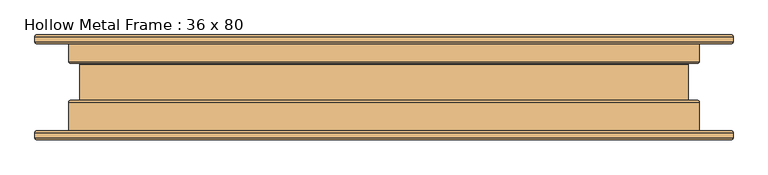
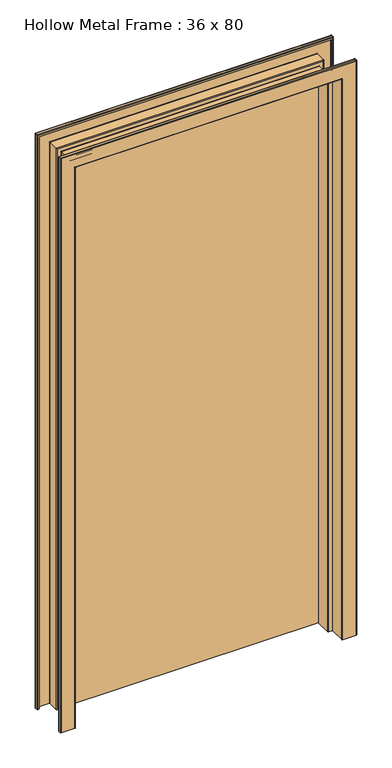
"""IFC4 building model written with IfcOpenShell, lengths in millimetres: door geometry, Hollow Metal Frame : 36 x 80."""

from ifc_helpers import new_model, si_unit, frame, origin, origin_with_axes, place, context, project, spatial, polyline, circle_curve, ellipse_curve, outline, extrude, source, transform, mapped, element, save
from ifc_brep_helpers import plane_surface, cylinder_surface, revolved_surface, advanced_brep


def hollow_metal_frame_36_x_80_ba635d64(model_context):
    return source(origin(), model_context, "Body", "SolidModel", [
        advanced_brep(
        [(-505.42825, -63.5635, 0.0), (-500.0625, -63.5635, 0.0), (-500.0625, -65.11925, 0.0), (-505.42825, -65.11925, 0.0), (-506.44425, -66.13525, 0.0), (-506.44425, -73.66, 0.0), (-505.42825, -74.676, 0.0), (-459.77175, -74.676, 0.0), (-458.75575, -73.66, 0.0), (-458.75575, -21.68525, 0.0), (-456.184, -19.1135, 0.0), (-443.89675, -19.1135, 0.0), (-442.88075, -18.0975, 0.0), (-442.88075, 33.6931, 0.0), (-443.89675, 34.7091, 0.0), (-456.184, 34.7091, 0.0), (-458.75575, 37.28085, 0.0), (-458.75575, 73.5965, 0.0), (-459.77175, 74.6125, 0.0), (-505.42825, 74.6125, 0.0), (-506.44425, 73.5965, 0.0), (-506.44425, 66.07175, 0.0), (-505.42825, 65.05575, 0.0), (-500.0625, 65.05575, 0.0), (-500.0625, 63.5, 0.0), (-505.42825, 63.5, 0.0), (-508.0, 66.07175, 0.0), (-508.0, 73.5965, 0.0), (-505.42825, 76.16825, 0.0), (-459.77175, 76.16825, 0.0), (-457.2, 73.5965, 0.0), (-457.2, 37.28085, 0.0), (-456.184, 36.26485, 0.0), (-443.89675, 36.26485, 0.0), (-441.325, 33.6931, 0.0), (-441.325, -18.0975, 0.0), (-443.89675, -20.66925, 0.0), (-456.184, -20.66925, 0.0), (-457.2, -21.68525, 0.0), (-457.2, -73.66, 0.0), (-459.77175, -76.23175, 0.0), (-505.42825, -76.23175, 0.0), (-508.0, -73.66, 0.0), (-508.0, -66.13525, 0.0), (-508.0, -66.13525, 2082.8000001), (-505.42825, -63.5635, 2080.2282501), (-508.0, -73.66, 2082.8000001), (-505.42825, -76.23175, 2080.2282501), (-459.77175, -76.23175, 2034.5717501), (459.77175, -76.23175, 2034.5717501), (459.77175, -76.23175, 0.0), (505.42825, -76.23175, 0.0), (505.42825, -76.23175, 2080.2282501), (-457.2, -73.66, 2032.0000001), (-457.2, -21.68525, 2032.0000001), (-456.184, -20.66925, 2030.9840001), (-443.89675, -20.66925, 2018.6967501), (443.89675, -20.66925, 2018.6967501), (443.89675, -20.66925, 0.0), (456.184, -20.66925, 0.0), (456.184, -20.66925, 2030.9840001), (-441.325, -18.0975, 2016.1250001), (-441.325, 33.6931, 2016.1250001), (-443.89675, 36.26485, 2018.6967501), (-456.184, 36.26485, 2030.9840001), (456.184, 36.26485, 2030.9840001), (456.184, 36.26485, 0.0), (443.89675, 36.26485, 0.0), (443.89675, 36.26485, 2018.6967501), (-457.2, 37.28085, 2032.0000001), (-457.2, 73.5965, 2032.0000001), (-459.77175, 76.16825, 2034.5717501), (-505.42825, 76.16825, 2080.2282501), (505.42825, 76.16825, 2080.2282501), (505.42825, 76.16825, 0.0), (459.77175, 76.16825, 0.0), (459.77175, 76.16825, 2034.5717501), (-508.0, 73.5965, 2082.8000001), (-508.0, 66.07175, 2082.8000001), (-505.42825, 63.5, 2080.2282501), (-500.0625, 63.5, 2074.8625001), (500.0625, 63.5, 2074.8625001), (500.0625, 63.5, 0.0), (505.42825, 63.5, 0.0), (505.42825, 63.5, 2080.2282501), (-500.0625, 65.05575, 2074.8625001), (-505.42825, 65.05575, 2080.2282501), (505.42825, 65.05575, 2080.2282501), (505.42825, 65.05575, 0.0), (500.0625, 65.05575, 0.0), (500.0625, 65.05575, 2074.8625001), (-506.44425, 66.07175, 2081.2442501), (-506.44425, 73.5965, 2081.2442501), (-505.42825, 74.6125, 2080.2282501), (-459.77175, 74.6125, 2034.5717501), (459.77175, 74.6125, 2034.5717501), (459.77175, 74.6125, 0.0), (505.42825, 74.6125, 0.0), (505.42825, 74.6125, 2080.2282501), (-458.75575, 73.5965, 2033.5557501), (-458.75575, 37.28085, 2033.5557501), (-456.184, 34.7091, 2030.9840001), (-443.89675, 34.7091, 2018.6967501), (443.89675, 34.7091, 2018.6967501), (443.89675, 34.7091, 0.0), (456.184, 34.7091, 0.0), (456.184, 34.7091, 2030.9840001), (-442.88075, 33.6931, 2017.6807501), (-442.88075, -18.0975, 2017.6807501), (-443.89675, -19.1135, 2018.6967501), (-456.184, -19.1135, 2030.9840001), (456.184, -19.1135, 2030.9840001), (456.184, -19.1135, 0.0), (443.89675, -19.1135, 0.0), (443.89675, -19.1135, 2018.6967501), (-458.75575, -21.68525, 2033.5557501), (-458.75575, -73.66, 2033.5557501), (-459.77175, -74.676, 2034.5717501), (-505.42825, -74.676, 2080.2282501), (505.42825, -74.676, 2080.2282501), (505.42825, -74.676, 0.0), (459.77175, -74.676, 0.0), (459.77175, -74.676, 2034.5717501), (-506.44425, -73.66, 2081.2442501), (-506.44425, -66.13525, 2081.2442501), (-505.42825, -65.11925, 2080.2282501), (-500.0625, -65.11925, 2074.8625001), (500.0625, -65.11925, 2074.8625001), (500.0625, -65.11925, 0.0), (505.42825, -65.11925, 0.0), (505.42825, -65.11925, 2080.2282501), (-500.0625, -63.5635, 2074.8625001), (505.42825, -63.5635, 2080.2282501), (505.42825, -63.5635, 0.0), (500.0625, -63.5635, 0.0), (500.0625, -63.5635, 2074.8625001), (508.0, -66.13525, 2082.8000001), (508.0, -73.66, 2082.8000001), (457.2, -73.66, 2032.0000001), (457.2, -21.68525, 2032.0000001), (441.325, -18.0975, 2016.1250001), (441.325, 33.6931, 2016.1250001), (457.2, 37.28085, 2032.0000001), (457.2, 73.5965, 2032.0000001), (508.0, 73.5965, 2082.8000001), (508.0, 66.07175, 2082.8000001), (506.44425, 66.07175, 2081.2442501), (506.44425, 73.5965, 2081.2442501), (458.75575, 73.5965, 2033.5557501), (458.75575, 37.28085, 2033.5557501), (442.88075, 33.6931, 2017.6807501), (442.88075, -18.0975, 2017.6807501), (458.75575, -21.68525, 2033.5557501), (458.75575, -73.66, 2033.5557501), (506.44425, -73.66, 2081.2442501), (506.44425, -66.13525, 2081.2442501), (508.0, -66.13525, 0.0), (508.0, -73.66, 0.0), (457.2, -73.66, 0.0), (457.2, -21.68525, 0.0), (441.325, -18.0975, 0.0), (441.325, 33.6931, 0.0), (457.2, 37.28085, 0.0), (457.2, 73.5965, 0.0), (508.0, 73.5965, 0.0), (508.0, 66.07175, 0.0), (506.44425, 66.07175, 0.0), (506.44425, 73.5965, 0.0), (458.75575, 73.5965, 0.0), (458.75575, 37.28085, 0.0), (442.88075, 33.6931, 0.0), (442.88075, -18.0975, 0.0), (458.75575, -21.68525, 0.0), (458.75575, -73.66, 0.0), (506.44425, -73.66, 0.0), (506.44425, -66.13525, 0.0)],
        [
            (0, 1),
            (1, 2),
            (2, 3),
            (3, 4, circle_curve(frame((-505.42825, -66.13525, 0.0), z_axis=(0.0, 0.0, 1.0), x_axis=(0.0, 1.0, 0.0)), 1.016)),
            (4, 5),
            (5, 6, circle_curve(frame((-505.42825, -73.66, 0.0), z_axis=(0.0, 0.0, 1.0), x_axis=(0.0, 1.0, 0.0)), 1.016)),
            (6, 7),
            (7, 8, circle_curve(frame((-459.77175, -73.66, 0.0), z_axis=(0.0, 0.0, 1.0), x_axis=(0.0, 1.0, 0.0)), 1.016)),
            (8, 9),
            (9, 10, circle_curve(frame((-456.184, -21.68525, 0.0), z_axis=(0.0, 0.0, -1.0), x_axis=(0.0, 1.0, 0.0)), 2.57175)),
            (10, 11),
            (11, 12, circle_curve(frame((-443.89675, -18.0975, 0.0), z_axis=(0.0, 0.0, 1.0), x_axis=(0.0, 1.0, 0.0)), 1.016)),
            (12, 13),
            (13, 14, circle_curve(frame((-443.89675, 33.6931, 0.0), z_axis=(0.0, 0.0, 1.0), x_axis=(0.0, 1.0, 0.0)), 1.016)),
            (14, 15),
            (15, 16, circle_curve(frame((-456.184, 37.28085, 0.0), z_axis=(0.0, 0.0, -1.0), x_axis=(0.0, 1.0, 0.0)), 2.57175)),
            (16, 17),
            (17, 18, circle_curve(frame((-459.77175, 73.5965, 0.0), z_axis=(0.0, 0.0, 1.0), x_axis=(0.0, 1.0, 0.0)), 1.016)),
            (18, 19),
            (19, 20, circle_curve(frame((-505.42825, 73.5965, 0.0), z_axis=(0.0, 0.0, 1.0), x_axis=(0.0, 1.0, 0.0)), 1.016)),
            (20, 21),
            (21, 22, circle_curve(frame((-505.42825, 66.07175, 0.0), z_axis=(0.0, 0.0, 1.0), x_axis=(0.0, 1.0, 0.0)), 1.016)),
            (22, 23),
            (23, 24),
            (24, 25),
            (25, 26, circle_curve(frame((-505.42825, 66.07175, 0.0), z_axis=(0.0, 0.0, -1.0), x_axis=(0.0, 1.0, 0.0)), 2.57175)),
            (26, 27),
            (27, 28, circle_curve(frame((-505.42825, 73.5965, 0.0), z_axis=(0.0, 0.0, -1.0), x_axis=(0.0, 1.0, 0.0)), 2.57175)),
            (28, 29),
            (29, 30, circle_curve(frame((-459.77175, 73.5965, 0.0), z_axis=(0.0, 0.0, -1.0), x_axis=(0.0, 1.0, 0.0)), 2.57175)),
            (30, 31),
            (31, 32, circle_curve(frame((-456.184, 37.28085, 0.0), z_axis=(0.0, 0.0, 1.0), x_axis=(0.0, 1.0, 0.0)), 1.016)),
            (32, 33),
            (33, 34, circle_curve(frame((-443.89675, 33.6931, 0.0), z_axis=(0.0, 0.0, -1.0), x_axis=(0.0, 1.0, 0.0)), 2.57175)),
            (34, 35),
            (35, 36, circle_curve(frame((-443.89675, -18.0975, 0.0), z_axis=(0.0, 0.0, -1.0), x_axis=(0.0, 1.0, 0.0)), 2.57175)),
            (36, 37),
            (37, 38, circle_curve(frame((-456.184, -21.68525, 0.0), z_axis=(0.0, 0.0, 1.0), x_axis=(0.0, 1.0, 0.0)), 1.016)),
            (38, 39),
            (39, 40, circle_curve(frame((-459.77175, -73.66, 0.0), z_axis=(0.0, 0.0, -1.0), x_axis=(0.0, 1.0, 0.0)), 2.57175)),
            (40, 41),
            (41, 42, circle_curve(frame((-505.42825, -73.66, 0.0), z_axis=(0.0, 0.0, -1.0), x_axis=(0.0, 1.0, 0.0)), 2.57175)),
            (42, 43),
            (43, 0, circle_curve(frame((-505.42825, -66.13525, 0.0), z_axis=(0.0, 0.0, -1.0), x_axis=(0.0, 1.0, 0.0)), 2.57175)),
            (43, 44),
            (44, 45, ellipse_curve(frame((-505.42825, -66.13525, 2080.2282501), z_axis=(-0.7071067811865475, 0.0, -0.7071067811865475), x_axis=(0.7071067811865474, 0.0, -0.7071067811865476)), 3.6370037, 2.57175)),
            (45, 0),
            (42, 46),
            (46, 44),
            (41, 47),
            (47, 46, ellipse_curve(frame((-505.42825, -73.66, 2080.2282501), z_axis=(-0.7071067811865475, 0.0, -0.7071067811865475), x_axis=(0.7071067811865474, 0.0, -0.7071067811865476)), 3.6370037, 2.57175)),
            (40, 48),
            (48, 49),
            (49, 50),
            (50, 51),
            (51, 52),
            (52, 47),
            (39, 53),
            (53, 48, ellipse_curve(frame((-459.77175, -73.66, 2034.5717501), z_axis=(-0.7071067811865475, 0.0, -0.7071067811865475), x_axis=(0.7071067811865474, 0.0, -0.7071067811865476)), 3.6370037, 2.57175)),
            (38, 54),
            (54, 53),
            (37, 55),
            (55, 54, ellipse_curve(frame((-456.184, -21.68525, 2030.9840001), z_axis=(0.7071067811865475, 0.0, 0.7071067811865475), x_axis=(-0.7071067811865474, 0.0, 0.7071067811865476)), 1.436841, 1.016)),
            (36, 56),
            (56, 57),
            (57, 58),
            (58, 59),
            (59, 60),
            (60, 55),
            (35, 61),
            (61, 56, ellipse_curve(frame((-443.89675, -18.0975, 2018.6967501), z_axis=(-0.7071067811865475, 0.0, -0.7071067811865475), x_axis=(0.7071067811865474, 0.0, -0.7071067811865476)), 3.6370037, 2.57175)),
            (34, 62),
            (62, 61),
            (33, 63),
            (63, 62, ellipse_curve(frame((-443.89675, 33.6931, 2018.6967501), z_axis=(-0.7071067811865475, 0.0, -0.7071067811865475), x_axis=(0.7071067811865474, 0.0, -0.7071067811865476)), 3.6370037, 2.57175)),
            (32, 64),
            (64, 65),
            (65, 66),
            (66, 67),
            (67, 68),
            (68, 63),
            (31, 69),
            (69, 64, ellipse_curve(frame((-456.184, 37.28085, 2030.9840001), z_axis=(0.7071067811865475, 0.0, 0.7071067811865475), x_axis=(-0.7071067811865474, 0.0, 0.7071067811865476)), 1.436841, 1.016)),
            (30, 70),
            (70, 69),
            (29, 71),
            (71, 70, ellipse_curve(frame((-459.77175, 73.5965, 2034.5717501), z_axis=(-0.7071067811865475, 0.0, -0.7071067811865475), x_axis=(0.7071067811865474, 0.0, -0.7071067811865476)), 3.6370037, 2.57175)),
            (28, 72),
            (72, 73),
            (73, 74),
            (74, 75),
            (75, 76),
            (76, 71),
            (27, 77),
            (77, 72, ellipse_curve(frame((-505.42825, 73.5965, 2080.2282501), z_axis=(-0.7071067811865475, 0.0, -0.7071067811865475), x_axis=(0.7071067811865474, 0.0, -0.7071067811865476)), 3.6370037, 2.57175)),
            (26, 78),
            (78, 77),
            (25, 79),
            (79, 78, ellipse_curve(frame((-505.42825, 66.07175, 2080.2282501), z_axis=(-0.7071067811865475, 0.0, -0.7071067811865475), x_axis=(0.7071067811865474, 0.0, -0.7071067811865476)), 3.6370037, 2.57175)),
            (24, 80),
            (80, 81),
            (81, 82),
            (82, 83),
            (83, 84),
            (84, 79),
            (23, 85),
            (85, 80),
            (22, 86),
            (86, 87),
            (87, 88),
            (88, 89),
            (89, 90),
            (90, 85),
            (21, 91),
            (91, 86, ellipse_curve(frame((-505.42825, 66.07175, 2080.2282501), z_axis=(0.7071067811865475, 0.0, 0.7071067811865475), x_axis=(-0.7071067811865474, 0.0, 0.7071067811865476)), 1.436841, 1.016)),
            (20, 92),
            (92, 91),
            (19, 93),
            (93, 92, ellipse_curve(frame((-505.42825, 73.5965, 2080.2282501), z_axis=(0.7071067811865475, 0.0, 0.7071067811865475), x_axis=(-0.7071067811865474, 0.0, 0.7071067811865476)), 1.436841, 1.016)),
            (18, 94),
            (94, 95),
            (95, 96),
            (96, 97),
            (97, 98),
            (98, 93),
            (17, 99),
            (99, 94, ellipse_curve(frame((-459.77175, 73.5965, 2034.5717501), z_axis=(0.7071067811865475, 0.0, 0.7071067811865475), x_axis=(-0.7071067811865474, 0.0, 0.7071067811865476)), 1.436841, 1.016)),
            (16, 100),
            (100, 99),
            (15, 101),
            (101, 100, ellipse_curve(frame((-456.184, 37.28085, 2030.9840001), z_axis=(-0.7071067811865475, 0.0, -0.7071067811865475), x_axis=(0.7071067811865474, 0.0, -0.7071067811865476)), 3.6370037, 2.57175)),
            (14, 102),
            (102, 103),
            (103, 104),
            (104, 105),
            (105, 106),
            (106, 101),
            (13, 107),
            (107, 102, ellipse_curve(frame((-443.89675, 33.6931, 2018.6967501), z_axis=(0.7071067811865475, 0.0, 0.7071067811865475), x_axis=(-0.7071067811865474, 0.0, 0.7071067811865476)), 1.436841, 1.016)),
            (12, 108),
            (108, 107),
            (11, 109),
            (109, 108, ellipse_curve(frame((-443.89675, -18.0975, 2018.6967501), z_axis=(0.7071067811865475, 0.0, 0.7071067811865475), x_axis=(-0.7071067811865474, 0.0, 0.7071067811865476)), 1.436841, 1.016)),
            (10, 110),
            (110, 111),
            (111, 112),
            (112, 113),
            (113, 114),
            (114, 109),
            (9, 115),
            (115, 110, ellipse_curve(frame((-456.184, -21.68525, 2030.9840001), z_axis=(-0.7071067811865475, 0.0, -0.7071067811865475), x_axis=(0.7071067811865474, 0.0, -0.7071067811865476)), 3.6370037, 2.57175)),
            (8, 116),
            (116, 115),
            (7, 117),
            (117, 116, ellipse_curve(frame((-459.77175, -73.66, 2034.5717501), z_axis=(0.7071067811865475, 0.0, 0.7071067811865475), x_axis=(-0.7071067811865474, 0.0, 0.7071067811865476)), 1.436841, 1.016)),
            (6, 118),
            (118, 119),
            (119, 120),
            (120, 121),
            (121, 122),
            (122, 117),
            (5, 123),
            (123, 118, ellipse_curve(frame((-505.42825, -73.66, 2080.2282501), z_axis=(0.7071067811865475, 0.0, 0.7071067811865475), x_axis=(-0.7071067811865474, 0.0, 0.7071067811865476)), 1.436841, 1.016)),
            (4, 124),
            (124, 123),
            (3, 125),
            (125, 124, ellipse_curve(frame((-505.42825, -66.13525, 2080.2282501), z_axis=(0.7071067811865475, 0.0, 0.7071067811865475), x_axis=(-0.7071067811865474, 0.0, 0.7071067811865476)), 1.436841, 1.016)),
            (2, 126),
            (126, 127),
            (127, 128),
            (128, 129),
            (129, 130),
            (130, 125),
            (1, 131),
            (131, 126),
            (45, 132),
            (132, 133),
            (133, 134),
            (134, 135),
            (135, 131),
            (44, 136),
            (136, 132, ellipse_curve(frame((505.42825, -66.13525, 2080.2282501), z_axis=(-0.7071067811865475, 0.0, 0.7071067811865475), x_axis=(-0.7071067811865476, 0.0, -0.7071067811865474)), 3.6370037, 2.57175)),
            (46, 137),
            (137, 136),
            (52, 137, ellipse_curve(frame((505.42825, -73.66, 2080.2282501), z_axis=(-0.7071067811865475, 0.0, 0.7071067811865475), x_axis=(-0.7071067811865476, 0.0, -0.7071067811865474)), 3.6370037, 2.57175)),
            (53, 138),
            (138, 49, ellipse_curve(frame((459.77175, -73.66, 2034.5717501), z_axis=(-0.7071067811865475, 0.0, 0.7071067811865475), x_axis=(-0.7071067811865476, 0.0, -0.7071067811865474)), 3.6370037, 2.57175)),
            (54, 139),
            (139, 138),
            (60, 139, ellipse_curve(frame((456.184, -21.68525, 2030.9840001), z_axis=(0.7071067811865475, 0.0, -0.7071067811865475), x_axis=(0.7071067811865476, 0.0, 0.7071067811865474)), 1.436841, 1.016)),
            (61, 140),
            (140, 57, ellipse_curve(frame((443.89675, -18.0975, 2018.6967501), z_axis=(-0.7071067811865475, 0.0, 0.7071067811865475), x_axis=(-0.7071067811865476, 0.0, -0.7071067811865474)), 3.6370037, 2.57175)),
            (62, 141),
            (141, 140),
            (68, 141, ellipse_curve(frame((443.89675, 33.6931, 2018.6967501), z_axis=(-0.7071067811865475, 0.0, 0.7071067811865475), x_axis=(-0.7071067811865476, 0.0, -0.7071067811865474)), 3.6370037, 2.57175)),
            (69, 142),
            (142, 65, ellipse_curve(frame((456.184, 37.28085, 2030.9840001), z_axis=(0.7071067811865475, 0.0, -0.7071067811865475), x_axis=(0.7071067811865476, 0.0, 0.7071067811865474)), 1.436841, 1.016)),
            (70, 143),
            (143, 142),
            (76, 143, ellipse_curve(frame((459.77175, 73.5965, 2034.5717501), z_axis=(-0.7071067811865475, 0.0, 0.7071067811865475), x_axis=(-0.7071067811865476, 0.0, -0.7071067811865474)), 3.6370037, 2.57175)),
            (77, 144),
            (144, 73, ellipse_curve(frame((505.42825, 73.5965, 2080.2282501), z_axis=(-0.7071067811865475, 0.0, 0.7071067811865475), x_axis=(-0.7071067811865476, 0.0, -0.7071067811865474)), 3.6370037, 2.57175)),
            (78, 145),
            (145, 144),
            (84, 145, ellipse_curve(frame((505.42825, 66.07175, 2080.2282501), z_axis=(-0.7071067811865475, 0.0, 0.7071067811865475), x_axis=(-0.7071067811865476, 0.0, -0.7071067811865474)), 3.6370037, 2.57175)),
            (90, 81),
            (91, 146),
            (146, 87, ellipse_curve(frame((505.42825, 66.07175, 2080.2282501), z_axis=(0.7071067811865475, 0.0, -0.7071067811865475), x_axis=(0.7071067811865476, 0.0, 0.7071067811865474)), 1.436841, 1.016)),
            (92, 147),
            (147, 146),
            (98, 147, ellipse_curve(frame((505.42825, 73.5965, 2080.2282501), z_axis=(0.7071067811865475, 0.0, -0.7071067811865475), x_axis=(0.7071067811865476, 0.0, 0.7071067811865474)), 1.436841, 1.016)),
            (99, 148),
            (148, 95, ellipse_curve(frame((459.77175, 73.5965, 2034.5717501), z_axis=(0.7071067811865475, 0.0, -0.7071067811865475), x_axis=(0.7071067811865476, 0.0, 0.7071067811865474)), 1.436841, 1.016)),
            (100, 149),
            (149, 148),
            (106, 149, ellipse_curve(frame((456.184, 37.28085, 2030.9840001), z_axis=(-0.7071067811865475, 0.0, 0.7071067811865475), x_axis=(-0.7071067811865476, 0.0, -0.7071067811865474)), 3.6370037, 2.57175)),
            (107, 150),
            (150, 103, ellipse_curve(frame((443.89675, 33.6931, 2018.6967501), z_axis=(0.7071067811865475, 0.0, -0.7071067811865475), x_axis=(0.7071067811865476, 0.0, 0.7071067811865474)), 1.436841, 1.016)),
            (108, 151),
            (151, 150),
            (114, 151, ellipse_curve(frame((443.89675, -18.0975, 2018.6967501), z_axis=(0.7071067811865475, 0.0, -0.7071067811865475), x_axis=(0.7071067811865476, 0.0, 0.7071067811865474)), 1.436841, 1.016)),
            (115, 152),
            (152, 111, ellipse_curve(frame((456.184, -21.68525, 2030.9840001), z_axis=(-0.7071067811865475, 0.0, 0.7071067811865475), x_axis=(-0.7071067811865476, 0.0, -0.7071067811865474)), 3.6370037, 2.57175)),
            (116, 153),
            (153, 152),
            (122, 153, ellipse_curve(frame((459.77175, -73.66, 2034.5717501), z_axis=(0.7071067811865475, 0.0, -0.7071067811865475), x_axis=(0.7071067811865476, 0.0, 0.7071067811865474)), 1.436841, 1.016)),
            (123, 154),
            (154, 119, ellipse_curve(frame((505.42825, -73.66, 2080.2282501), z_axis=(0.7071067811865475, 0.0, -0.7071067811865475), x_axis=(0.7071067811865476, 0.0, 0.7071067811865474)), 1.436841, 1.016)),
            (124, 155),
            (155, 154),
            (130, 155, ellipse_curve(frame((505.42825, -66.13525, 2080.2282501), z_axis=(0.7071067811865475, 0.0, -0.7071067811865475), x_axis=(0.7071067811865476, 0.0, 0.7071067811865474)), 1.436841, 1.016)),
            (135, 127),
            (133, 156, circle_curve(frame((505.42825, -66.13525, 0.0), z_axis=(0.0, 0.0, -1.0), x_axis=(0.0, 1.0, 0.0)), 2.57175)),
            (156, 157),
            (157, 51, circle_curve(frame((505.42825, -73.66, 0.0), z_axis=(0.0, 0.0, -1.0), x_axis=(0.0, 1.0, 0.0)), 2.57175)),
            (50, 158, circle_curve(frame((459.77175, -73.66, 0.0), z_axis=(0.0, 0.0, -1.0), x_axis=(0.0, 1.0, 0.0)), 2.57175)),
            (158, 159),
            (159, 59, circle_curve(frame((456.184, -21.68525, 0.0), z_axis=(0.0, 0.0, 1.0), x_axis=(0.0, 1.0, 0.0)), 1.016)),
            (58, 160, circle_curve(frame((443.89675, -18.0975, 0.0), z_axis=(0.0, 0.0, -1.0), x_axis=(0.0, 1.0, 0.0)), 2.57175)),
            (160, 161),
            (161, 67, circle_curve(frame((443.89675, 33.6931, 0.0), z_axis=(0.0, 0.0, -1.0), x_axis=(0.0, 1.0, 0.0)), 2.57175)),
            (66, 162, circle_curve(frame((456.184, 37.28085, 0.0), z_axis=(0.0, 0.0, 1.0), x_axis=(0.0, 1.0, 0.0)), 1.016)),
            (162, 163),
            (163, 75, circle_curve(frame((459.77175, 73.5965, 0.0), z_axis=(0.0, 0.0, -1.0), x_axis=(0.0, 1.0, 0.0)), 2.57175)),
            (74, 164, circle_curve(frame((505.42825, 73.5965, 0.0), z_axis=(0.0, 0.0, -1.0), x_axis=(0.0, 1.0, 0.0)), 2.57175)),
            (164, 165),
            (165, 83, circle_curve(frame((505.42825, 66.07175, 0.0), z_axis=(0.0, 0.0, -1.0), x_axis=(0.0, 1.0, 0.0)), 2.57175)),
            (82, 89),
            (88, 166, circle_curve(frame((505.42825, 66.07175, 0.0), z_axis=(0.0, 0.0, 1.0), x_axis=(0.0, 1.0, 0.0)), 1.016)),
            (166, 167),
            (167, 97, circle_curve(frame((505.42825, 73.5965, 0.0), z_axis=(0.0, 0.0, 1.0), x_axis=(0.0, 1.0, 0.0)), 1.016)),
            (96, 168, circle_curve(frame((459.77175, 73.5965, 0.0), z_axis=(0.0, 0.0, 1.0), x_axis=(0.0, 1.0, 0.0)), 1.016)),
            (168, 169),
            (169, 105, circle_curve(frame((456.184, 37.28085, 0.0), z_axis=(0.0, 0.0, -1.0), x_axis=(0.0, 1.0, 0.0)), 2.57175)),
            (104, 170, circle_curve(frame((443.89675, 33.6931, 0.0), z_axis=(0.0, 0.0, 1.0), x_axis=(0.0, 1.0, 0.0)), 1.016)),
            (170, 171),
            (171, 113, circle_curve(frame((443.89675, -18.0975, 0.0), z_axis=(0.0, 0.0, 1.0), x_axis=(0.0, 1.0, 0.0)), 1.016)),
            (112, 172, circle_curve(frame((456.184, -21.68525, 0.0), z_axis=(0.0, 0.0, -1.0), x_axis=(0.0, 1.0, 0.0)), 2.57175)),
            (172, 173),
            (173, 121, circle_curve(frame((459.77175, -73.66, 0.0), z_axis=(0.0, 0.0, 1.0), x_axis=(0.0, 1.0, 0.0)), 1.016)),
            (120, 174, circle_curve(frame((505.42825, -73.66, 0.0), z_axis=(0.0, 0.0, 1.0), x_axis=(0.0, 1.0, 0.0)), 1.016)),
            (174, 175),
            (175, 129, circle_curve(frame((505.42825, -66.13525, 0.0), z_axis=(0.0, 0.0, 1.0), x_axis=(0.0, 1.0, 0.0)), 1.016)),
            (128, 134),
            (136, 156),
            (137, 157),
            (138, 158),
            (139, 159),
            (140, 160),
            (141, 161),
            (142, 162),
            (143, 163),
            (144, 164),
            (145, 165),
            (146, 166),
            (147, 167),
            (148, 168),
            (149, 169),
            (150, 170),
            (151, 171),
            (152, 172),
            (153, 173),
            (154, 174),
            (155, 175),
        ],
        [
            plane_surface(frame((-468.3125, 63.5, 0.0), z_axis=(0.0, 0.0, -1.0), x_axis=(1.0, 0.0, 0.0))),
            cylinder_surface(frame((-505.42825, -66.13525, 0.0), z_axis=(0.0, 0.0, -1.0), x_axis=(0.0, 1.0, 0.0)), 2.57175),
            plane_surface(frame((-508.0, -66.13525, 0.0), z_axis=(-1.0, 0.0, 0.0), x_axis=(0.0, 0.0, 1.0))),
            cylinder_surface(frame((-505.42825, -73.66, 0.0), z_axis=(0.0, 0.0, -1.0), x_axis=(0.0, 1.0, 0.0)), 2.57175),
            plane_surface(frame((-505.42825, -76.23175, 0.0), z_axis=(0.0, -1.0, 0.0), x_axis=(0.0, 0.0, 1.0))),
            cylinder_surface(frame((-459.77175, -73.66, 0.0), z_axis=(0.0, 0.0, -1.0), x_axis=(0.0, 1.0, 0.0)), 2.57175),
            plane_surface(frame((-457.2, -73.66, 0.0), z_axis=(1.0, 0.0, 0.0), x_axis=(0.0, 0.0, 1.0))),
            revolved_surface(polyline([(-456.184, -20.669249999999998, 2032.0000001145868), (-456.184, -20.669249999999998, 0.0)]), (-456.184, -21.68525, 0.0), (0.0, 0.0, 1.0)),
            plane_surface(frame((-456.184, -20.66925, 0.0), z_axis=(0.0, -1.0, 0.0), x_axis=(0.0, 0.0, 1.0))),
            cylinder_surface(frame((-443.89675, -18.0975, 0.0), z_axis=(0.0, 0.0, -1.0), x_axis=(0.0, 1.0, 0.0)), 2.57175),
            plane_surface(frame((-441.325, -18.0975, 0.0), z_axis=(1.0, 0.0, 0.0), x_axis=(0.0, 0.0, 1.0))),
            cylinder_surface(frame((-443.89675, 33.6931, 0.0), z_axis=(0.0, 0.0, -1.0), x_axis=(0.0, 1.0, 0.0)), 2.57175),
            plane_surface(frame((-443.89675, 36.26485, 0.0), z_axis=(0.0, 1.0, 0.0), x_axis=(0.0, 0.0, 1.0))),
            revolved_surface(polyline([(-456.184, 38.29685, 2032.0000001145868), (-456.184, 38.29685, 0.0)]), (-456.184, 37.28085, 0.0), (0.0, 0.0, 1.0)),
            plane_surface(frame((-457.2, 37.28085, 0.0), z_axis=(1.0, 0.0, 0.0), x_axis=(0.0, 0.0, 1.0))),
            cylinder_surface(frame((-459.77175, 73.5965, 0.0), z_axis=(0.0, 0.0, -1.0), x_axis=(0.0, 1.0, 0.0)), 2.57175),
            plane_surface(frame((-459.77175, 76.16825, 0.0), z_axis=(0.0, 1.0, 0.0), x_axis=(0.0, 0.0, 1.0))),
            cylinder_surface(frame((-505.42825, 73.5965, 0.0), z_axis=(0.0, 0.0, -1.0), x_axis=(0.0, 1.0, 0.0)), 2.57175),
            plane_surface(frame((-508.0, 73.5965, 0.0), z_axis=(-1.0, 0.0, 0.0), x_axis=(0.0, 0.0, 1.0))),
            cylinder_surface(frame((-505.42825, 66.07175, 0.0), z_axis=(0.0, 0.0, -1.0), x_axis=(0.0, 1.0, 0.0)), 2.57175),
            plane_surface(frame((-505.42825, 63.5, 0.0), z_axis=(0.0, -1.0, 0.0), x_axis=(0.0, 0.0, 1.0))),
            plane_surface(frame((-500.0625, 63.5, 0.0), z_axis=(1.0, 0.0, 0.0), x_axis=(0.0, 0.0, 1.0))),
            plane_surface(frame((-500.0625, 65.05575, 0.0), z_axis=(0.0, 1.0, 0.0), x_axis=(0.0, 0.0, 1.0))),
            revolved_surface(polyline([(-505.42825, 67.08775, 2081.244250114587), (-505.42825, 67.08775, 0.0)]), (-505.42825, 66.07175, 0.0), (0.0, 0.0, 1.0)),
            plane_surface(frame((-506.44425, 66.07175, 0.0), z_axis=(1.0, 0.0, 0.0), x_axis=(0.0, 0.0, 1.0))),
            revolved_surface(polyline([(-505.42825, 74.61250000000001, 2081.244250114587), (-505.42825, 74.61250000000001, 0.0)]), (-505.42825, 73.5965, 0.0), (0.0, 0.0, 1.0)),
            plane_surface(frame((-505.42825, 74.6125, 0.0), z_axis=(0.0, -1.0, 0.0), x_axis=(0.0, 0.0, 1.0))),
            revolved_surface(polyline([(-459.77175, 74.61250000000001, 2035.5877501145867), (-459.77175, 74.61250000000001, 0.0)]), (-459.77175, 73.5965, 0.0), (0.0, 0.0, 1.0)),
            plane_surface(frame((-458.75575, 73.5965, 0.0), z_axis=(-1.0, 0.0, 0.0), x_axis=(0.0, 0.0, 1.0))),
            cylinder_surface(frame((-456.184, 37.28085, 0.0), z_axis=(0.0, 0.0, -1.0), x_axis=(0.0, 1.0, 0.0)), 2.57175),
            plane_surface(frame((-456.184, 34.7091, 0.0), z_axis=(0.0, -1.0, 0.0), x_axis=(0.0, 0.0, 1.0))),
            revolved_surface(polyline([(-443.89675, 34.7091, 2019.7127501145867), (-443.89675, 34.7091, 0.0)]), (-443.89675, 33.6931, 0.0), (0.0, 0.0, 1.0)),
            plane_surface(frame((-442.88075, 33.6931, 0.0), z_axis=(-1.0, 0.0, 0.0), x_axis=(0.0, 0.0, 1.0))),
            revolved_surface(polyline([(-443.89675, -17.0815, 2019.7127501145867), (-443.89675, -17.0815, 0.0)]), (-443.89675, -18.0975, 0.0), (0.0, 0.0, 1.0)),
            plane_surface(frame((-443.89675, -19.1135, 0.0), z_axis=(0.0, 1.0, 0.0), x_axis=(0.0, 0.0, 1.0))),
            cylinder_surface(frame((-456.184, -21.68525, 0.0), z_axis=(0.0, 0.0, -1.0), x_axis=(0.0, 1.0, 0.0)), 2.57175),
            plane_surface(frame((-458.75575, -21.68525, 0.0), z_axis=(-1.0, 0.0, 0.0), x_axis=(0.0, 0.0, 1.0))),
            revolved_surface(polyline([(-459.77175, -72.64399999999999, 2035.5877501145867), (-459.77175, -72.64399999999999, 0.0)]), (-459.77175, -73.66, 0.0), (0.0, 0.0, 1.0)),
            plane_surface(frame((-459.77175, -74.676, 0.0), z_axis=(0.0, 1.0, 0.0), x_axis=(0.0, 0.0, 1.0))),
            revolved_surface(polyline([(-505.42825, -72.64399999999999, 2081.244250114587), (-505.42825, -72.64399999999999, 0.0)]), (-505.42825, -73.66, 0.0), (0.0, 0.0, 1.0)),
            plane_surface(frame((-506.44425, -73.66, 0.0), z_axis=(1.0, 0.0, 0.0), x_axis=(0.0, 0.0, 1.0))),
            revolved_surface(polyline([(-505.42825, -65.11925, 2081.244250114587), (-505.42825, -65.11925, 0.0)]), (-505.42825, -66.13525, 0.0), (0.0, 0.0, 1.0)),
            plane_surface(frame((-505.42825, -65.11925, 0.0), z_axis=(0.0, -1.0, 0.0), x_axis=(0.0, 0.0, 1.0))),
            plane_surface(frame((-500.0625, -65.11925, 0.0), z_axis=(1.0, 0.0, 0.0), x_axis=(0.0, 0.0, 1.0))),
            plane_surface(frame((-500.0625, -63.5635, 0.0), z_axis=(0.0, 1.0, 0.0), x_axis=(0.0, 0.0, 1.0))),
            cylinder_surface(frame((-468.3125, -66.13525, 2080.2282501), z_axis=(-1.0, 0.0, 0.0), x_axis=(0.0, 1.0, 0.0)), 2.57175),
            plane_surface(frame((-508.0, -66.13525, 2082.8000001), z_axis=(0.0, 0.0, 1.0), x_axis=(1.0, 0.0, 0.0))),
            cylinder_surface(frame((-468.3125, -73.66, 2080.2282501), z_axis=(-1.0, 0.0, 0.0), x_axis=(0.0, 1.0, 0.0)), 2.57175),
            cylinder_surface(frame((-468.3125, -73.66, 2034.5717501), z_axis=(-1.0, 0.0, 0.0), x_axis=(0.0, 1.0, 0.0)), 2.57175),
            plane_surface(frame((-457.2, -73.66, 2032.0000001), z_axis=(0.0, 0.0, -1.0), x_axis=(1.0, 0.0, 0.0))),
            revolved_surface(polyline([(457.20000001458686, -20.669249999999998, 2030.9840001), (-457.20000001458686, -20.669249999999998, 2030.9840001)]), (-468.3125, -21.68525, 2030.9840001), (1.0, 0.0, 0.0)),
            cylinder_surface(frame((-468.3125, -18.0975, 2018.6967501), z_axis=(-1.0, 0.0, 0.0), x_axis=(0.0, 1.0, 0.0)), 2.57175),
            plane_surface(frame((-441.325, -18.0975, 2016.1250001), z_axis=(0.0, 0.0, -1.0), x_axis=(1.0, 0.0, 0.0))),
            cylinder_surface(frame((-468.3125, 33.6931, 2018.6967501), z_axis=(-1.0, 0.0, 0.0), x_axis=(0.0, 1.0, 0.0)), 2.57175),
            revolved_surface(polyline([(457.20000001458686, 38.29685, 2030.9840001), (-457.20000001458686, 38.29685, 2030.9840001)]), (-468.3125, 37.28085, 2030.9840001), (1.0, 0.0, 0.0)),
            plane_surface(frame((-457.2, 37.28085, 2032.0000001), z_axis=(0.0, 0.0, -1.0), x_axis=(1.0, 0.0, 0.0))),
            cylinder_surface(frame((-468.3125, 73.5965, 2034.5717501), z_axis=(-1.0, 0.0, 0.0), x_axis=(0.0, 1.0, 0.0)), 2.57175),
            cylinder_surface(frame((-468.3125, 73.5965, 2080.2282501), z_axis=(-1.0, 0.0, 0.0), x_axis=(0.0, 1.0, 0.0)), 2.57175),
            plane_surface(frame((-508.0, 73.5965, 2082.8000001), z_axis=(0.0, 0.0, 1.0), x_axis=(1.0, 0.0, 0.0))),
            cylinder_surface(frame((-468.3125, 66.07175, 2080.2282501), z_axis=(-1.0, 0.0, 0.0), x_axis=(0.0, 1.0, 0.0)), 2.57175),
            plane_surface(frame((-500.0625, 63.5, 2074.8625001), z_axis=(0.0, 0.0, -1.0), x_axis=(1.0, 0.0, 0.0))),
            revolved_surface(polyline([(506.4442500145868, 67.08775, 2080.2282501), (-506.4442500145868, 67.08775, 2080.2282501)]), (-468.3125, 66.07175, 2080.2282501), (1.0, 0.0, 0.0)),
            plane_surface(frame((-506.44425, 66.07175, 2081.2442501), z_axis=(0.0, 0.0, -1.0), x_axis=(1.0, 0.0, 0.0))),
            revolved_surface(polyline([(506.4442500145868, 74.61250000000001, 2080.2282501), (-506.4442500145868, 74.61250000000001, 2080.2282501)]), (-468.3125, 73.5965, 2080.2282501), (1.0, 0.0, 0.0)),
            revolved_surface(polyline([(460.7877500145869, 74.61250000000001, 2034.5717501), (-460.78775001458683, 74.61250000000001, 2034.5717501)]), (-468.3125, 73.5965, 2034.5717501), (1.0, 0.0, 0.0)),
            plane_surface(frame((-458.75575, 73.5965, 2033.5557501), z_axis=(0.0, 0.0, 1.0), x_axis=(1.0, 0.0, 0.0))),
            cylinder_surface(frame((-468.3125, 37.28085, 2030.9840001), z_axis=(-1.0, 0.0, 0.0), x_axis=(0.0, 1.0, 0.0)), 2.57175),
            revolved_surface(polyline([(444.9127500145869, 34.7091, 2018.6967501), (-444.91275001458683, 34.7091, 2018.6967501)]), (-468.3125, 33.6931, 2018.6967501), (1.0, 0.0, 0.0)),
            plane_surface(frame((-442.88075, 33.6931, 2017.6807501), z_axis=(0.0, 0.0, 1.0), x_axis=(1.0, 0.0, 0.0))),
            revolved_surface(polyline([(444.9127500145869, -17.0815, 2018.6967501), (-444.91275001458683, -17.0815, 2018.6967501)]), (-468.3125, -18.0975, 2018.6967501), (1.0, 0.0, 0.0)),
            cylinder_surface(frame((-468.3125, -21.68525, 2030.9840001), z_axis=(-1.0, 0.0, 0.0), x_axis=(0.0, 1.0, 0.0)), 2.57175),
            plane_surface(frame((-458.75575, -21.68525, 2033.5557501), z_axis=(0.0, 0.0, 1.0), x_axis=(1.0, 0.0, 0.0))),
            revolved_surface(polyline([(460.7877500145869, -72.64399999999999, 2034.5717501), (-460.78775001458683, -72.64399999999999, 2034.5717501)]), (-468.3125, -73.66, 2034.5717501), (1.0, 0.0, 0.0)),
            revolved_surface(polyline([(506.4442500145868, -72.64399999999999, 2080.2282501), (-506.4442500145868, -72.64399999999999, 2080.2282501)]), (-468.3125, -73.66, 2080.2282501), (1.0, 0.0, 0.0)),
            plane_surface(frame((-506.44425, -73.66, 2081.2442501), z_axis=(0.0, 0.0, -1.0), x_axis=(1.0, 0.0, 0.0))),
            revolved_surface(polyline([(506.4442500145868, -65.11925, 2080.2282501), (-506.4442500145868, -65.11925, 2080.2282501)]), (-468.3125, -66.13525, 2080.2282501), (1.0, 0.0, 0.0)),
            plane_surface(frame((-500.0625, -65.11925, 2074.8625001), z_axis=(0.0, 0.0, -1.0), x_axis=(1.0, 0.0, 0.0))),
            plane_surface(frame((468.3125, 63.5, 0.0), z_axis=(0.0, 0.0, -1.0), x_axis=(-1.0, 0.0, 0.0))),
            cylinder_surface(frame((505.42825, -66.13525, 2043.1125001), z_axis=(0.0, 0.0, 1.0), x_axis=(0.0, 1.0, 0.0)), 2.57175),
            plane_surface(frame((508.0, -66.13525, 2082.8000001), z_axis=(1.0, 0.0, 0.0), x_axis=(0.0, 0.0, -1.0))),
            cylinder_surface(frame((505.42825, -73.66, 2043.1125001), z_axis=(0.0, 0.0, 1.0), x_axis=(0.0, 1.0, 0.0)), 2.57175),
            cylinder_surface(frame((459.77175, -73.66, 2043.1125001), z_axis=(0.0, 0.0, 1.0), x_axis=(0.0, 1.0, 0.0)), 2.57175),
            plane_surface(frame((457.2, -73.66, 2032.0000001), z_axis=(-1.0, 0.0, 0.0), x_axis=(0.0, 0.0, -1.0))),
            revolved_surface(polyline([(456.184, -20.669249999999998, 0.0), (456.184, -20.669249999999998, 2032.0000001145868)]), (456.184, -21.68525, 2043.1125001), (0.0, 0.0, -1.0)),
            cylinder_surface(frame((443.89675, -18.0975, 2043.1125001), z_axis=(0.0, 0.0, 1.0), x_axis=(0.0, 1.0, 0.0)), 2.57175),
            plane_surface(frame((441.325, -18.0975, 2016.1250001), z_axis=(-1.0, 0.0, 0.0), x_axis=(0.0, 0.0, -1.0))),
            cylinder_surface(frame((443.89675, 33.6931, 2043.1125001), z_axis=(0.0, 0.0, 1.0), x_axis=(0.0, 1.0, 0.0)), 2.57175),
            revolved_surface(polyline([(456.184, 38.29685, 0.0), (456.184, 38.29685, 2032.0000001145868)]), (456.184, 37.28085, 2043.1125001), (0.0, 0.0, -1.0)),
            plane_surface(frame((457.2, 37.28085, 2032.0000001), z_axis=(-1.0, 0.0, 0.0), x_axis=(0.0, 0.0, -1.0))),
            cylinder_surface(frame((459.77175, 73.5965, 2043.1125001), z_axis=(0.0, 0.0, 1.0), x_axis=(0.0, 1.0, 0.0)), 2.57175),
            cylinder_surface(frame((505.42825, 73.5965, 2043.1125001), z_axis=(0.0, 0.0, 1.0), x_axis=(0.0, 1.0, 0.0)), 2.57175),
            plane_surface(frame((508.0, 73.5965, 2082.8000001), z_axis=(1.0, 0.0, 0.0), x_axis=(0.0, 0.0, -1.0))),
            cylinder_surface(frame((505.42825, 66.07175, 2043.1125001), z_axis=(0.0, 0.0, 1.0), x_axis=(0.0, 1.0, 0.0)), 2.57175),
            plane_surface(frame((500.0625, 63.5, 2074.8625001), z_axis=(-1.0, 0.0, 0.0), x_axis=(0.0, 0.0, -1.0))),
            revolved_surface(polyline([(505.42825, 67.08775, 0.0), (505.42825, 67.08775, 2081.244250114587)]), (505.42825, 66.07175, 2043.1125001), (0.0, 0.0, -1.0)),
            plane_surface(frame((506.44425, 66.07175, 2081.2442501), z_axis=(-1.0, 0.0, 0.0), x_axis=(0.0, 0.0, -1.0))),
            revolved_surface(polyline([(505.42825, 74.61250000000001, 0.0), (505.42825, 74.61250000000001, 2081.244250114587)]), (505.42825, 73.5965, 2043.1125001), (0.0, 0.0, -1.0)),
            revolved_surface(polyline([(459.77175, 74.61250000000001, 0.0), (459.77175, 74.61250000000001, 2035.5877501145867)]), (459.77175, 73.5965, 2043.1125001), (0.0, 0.0, -1.0)),
            plane_surface(frame((458.75575, 73.5965, 2033.5557501), z_axis=(1.0, 0.0, 0.0), x_axis=(0.0, 0.0, -1.0))),
            cylinder_surface(frame((456.184, 37.28085, 2043.1125001), z_axis=(0.0, 0.0, 1.0), x_axis=(0.0, 1.0, 0.0)), 2.57175),
            revolved_surface(polyline([(443.89675, 34.7091, 0.0), (443.89675, 34.7091, 2019.7127501145867)]), (443.89675, 33.6931, 2043.1125001), (0.0, 0.0, -1.0)),
            plane_surface(frame((442.88075, 33.6931, 2017.6807501), z_axis=(1.0, 0.0, 0.0), x_axis=(0.0, 0.0, -1.0))),
            revolved_surface(polyline([(443.89675, -17.0815, 0.0), (443.89675, -17.0815, 2019.7127501145867)]), (443.89675, -18.0975, 2043.1125001), (0.0, 0.0, -1.0)),
            cylinder_surface(frame((456.184, -21.68525, 2043.1125001), z_axis=(0.0, 0.0, 1.0), x_axis=(0.0, 1.0, 0.0)), 2.57175),
            plane_surface(frame((458.75575, -21.68525, 2033.5557501), z_axis=(1.0, 0.0, 0.0), x_axis=(0.0, 0.0, -1.0))),
            revolved_surface(polyline([(459.77175, -72.64399999999999, 0.0), (459.77175, -72.64399999999999, 2035.5877501145867)]), (459.77175, -73.66, 2043.1125001), (0.0, 0.0, -1.0)),
            revolved_surface(polyline([(505.42825, -72.64399999999999, 0.0), (505.42825, -72.64399999999999, 2081.244250114587)]), (505.42825, -73.66, 2043.1125001), (0.0, 0.0, -1.0)),
            plane_surface(frame((506.44425, -73.66, 2081.2442501), z_axis=(-1.0, 0.0, 0.0), x_axis=(0.0, 0.0, -1.0))),
            revolved_surface(polyline([(505.42825, -65.11925, 0.0), (505.42825, -65.11925, 2081.244250114587)]), (505.42825, -66.13525, 2043.1125001), (0.0, 0.0, -1.0)),
            plane_surface(frame((500.0625, -65.11925, 2074.8625001), z_axis=(-1.0, 0.0, 0.0), x_axis=(0.0, 0.0, -1.0))),
        ],
        [
            (0, [[1, 2, 3, 4, 5, 6, 7, 8, 9, 10, 11, 12, 13, 14, 15, 16, 17, 18, 19, 20, 21, 22, 23, 24, 25, 26, 27, 28, 29, 30, 31, 32, 33, 34, 35, 36, 37, 38, 39, 40, 41, 42, 43, 44]]),
            (1, [[45, 46, 47, -44]]),
            (2, [[48, 49, -45, -43]]),
            (3, [[50, 51, -48, -42]]),
            (4, [[52, 53, 54, 55, 56, 57, -50, -41]]),
            (5, [[58, 59, -52, -40]]),
            (6, [[60, 61, -58, -39]]),
            (7, [[62, 63, -60, -38]]),
            (8, [[64, 65, 66, 67, 68, 69, -62, -37]]),
            (9, [[70, 71, -64, -36]]),
            (10, [[72, 73, -70, -35]]),
            (11, [[74, 75, -72, -34]]),
            (12, [[76, 77, 78, 79, 80, 81, -74, -33]]),
            (13, [[82, 83, -76, -32]]),
            (14, [[84, 85, -82, -31]]),
            (15, [[86, 87, -84, -30]]),
            (16, [[88, 89, 90, 91, 92, 93, -86, -29]]),
            (17, [[94, 95, -88, -28]]),
            (18, [[96, 97, -94, -27]]),
            (19, [[98, 99, -96, -26]]),
            (20, [[100, 101, 102, 103, 104, 105, -98, -25]]),
            (21, [[106, 107, -100, -24]]),
            (22, [[108, 109, 110, 111, 112, 113, -106, -23]]),
            (23, [[114, 115, -108, -22]]),
            (24, [[116, 117, -114, -21]]),
            (25, [[118, 119, -116, -20]]),
            (26, [[120, 121, 122, 123, 124, 125, -118, -19]]),
            (27, [[126, 127, -120, -18]]),
            (28, [[128, 129, -126, -17]]),
            (29, [[130, 131, -128, -16]]),
            (30, [[132, 133, 134, 135, 136, 137, -130, -15]]),
            (31, [[138, 139, -132, -14]]),
            (32, [[140, 141, -138, -13]]),
            (33, [[142, 143, -140, -12]]),
            (34, [[144, 145, 146, 147, 148, 149, -142, -11]]),
            (35, [[150, 151, -144, -10]]),
            (36, [[152, 153, -150, -9]]),
            (37, [[154, 155, -152, -8]]),
            (38, [[156, 157, 158, 159, 160, 161, -154, -7]]),
            (39, [[162, 163, -156, -6]]),
            (40, [[164, 165, -162, -5]]),
            (41, [[166, 167, -164, -4]]),
            (42, [[168, 169, 170, 171, 172, 173, -166, -3]]),
            (43, [[174, 175, -168, -2]]),
            (44, [[-47, 176, 177, 178, 179, 180, -174, -1]]),
            (45, [[181, 182, -176, -46]]),
            (46, [[183, 184, -181, -49]]),
            (47, [[-57, 185, -183, -51]]),
            (48, [[186, 187, -53, -59]]),
            (49, [[188, 189, -186, -61]]),
            (50, [[-69, 190, -188, -63]]),
            (51, [[191, 192, -65, -71]]),
            (52, [[193, 194, -191, -73]]),
            (53, [[-81, 195, -193, -75]]),
            (54, [[196, 197, -77, -83]]),
            (55, [[198, 199, -196, -85]]),
            (56, [[-93, 200, -198, -87]]),
            (57, [[201, 202, -89, -95]]),
            (58, [[203, 204, -201, -97]]),
            (59, [[-105, 205, -203, -99]]),
            (60, [[-113, 206, -101, -107]]),
            (61, [[207, 208, -109, -115]]),
            (62, [[209, 210, -207, -117]]),
            (63, [[-125, 211, -209, -119]]),
            (64, [[212, 213, -121, -127]]),
            (65, [[214, 215, -212, -129]]),
            (66, [[-137, 216, -214, -131]]),
            (67, [[217, 218, -133, -139]]),
            (68, [[219, 220, -217, -141]]),
            (69, [[-149, 221, -219, -143]]),
            (70, [[222, 223, -145, -151]]),
            (71, [[224, 225, -222, -153]]),
            (72, [[-161, 226, -224, -155]]),
            (73, [[227, 228, -157, -163]]),
            (74, [[229, 230, -227, -165]]),
            (75, [[-173, 231, -229, -167]]),
            (76, [[-180, 232, -169, -175]]),
            (77, [[233, 234, 235, -55, 236, 237, 238, -67, 239, 240, 241, -79, 242, 243, 244, -91, 245, 246, 247, -103, 248, -111, 249, 250, 251, -123, 252, 253, 254, -135, 255, 256, 257, -147, 258, 259, 260, -159, 261, 262, 263, -171, 264, -178]]),
            (78, [[265, -233, -177, -182]]),
            (79, [[266, -234, -265, -184]]),
            (80, [[-56, -235, -266, -185]]),
            (81, [[267, -236, -54, -187]]),
            (82, [[268, -237, -267, -189]]),
            (83, [[-68, -238, -268, -190]]),
            (84, [[269, -239, -66, -192]]),
            (85, [[270, -240, -269, -194]]),
            (86, [[-80, -241, -270, -195]]),
            (87, [[271, -242, -78, -197]]),
            (88, [[272, -243, -271, -199]]),
            (89, [[-92, -244, -272, -200]]),
            (90, [[273, -245, -90, -202]]),
            (91, [[274, -246, -273, -204]]),
            (92, [[-104, -247, -274, -205]]),
            (93, [[-112, -248, -102, -206]]),
            (94, [[275, -249, -110, -208]]),
            (95, [[276, -250, -275, -210]]),
            (96, [[-124, -251, -276, -211]]),
            (97, [[277, -252, -122, -213]]),
            (98, [[278, -253, -277, -215]]),
            (99, [[-136, -254, -278, -216]]),
            (100, [[279, -255, -134, -218]]),
            (101, [[280, -256, -279, -220]]),
            (102, [[-148, -257, -280, -221]]),
            (103, [[281, -258, -146, -223]]),
            (104, [[282, -259, -281, -225]]),
            (105, [[-160, -260, -282, -226]]),
            (106, [[283, -261, -158, -228]]),
            (107, [[284, -262, -283, -230]]),
            (108, [[-172, -263, -284, -231]]),
            (109, [[-179, -264, -170, -232]]),
        ],
    ),
        extrude(outline(polyline([(455.64425, 37.28085), (-455.64425, 37.28085), (-455.64425, 63.5), (455.64425, 63.5), (455.64425, 37.28085)])), origin_with_axes(), (0.0, 0.0, 1.0), 2032.0000001),
    ])


if __name__ == "__main__":
    model = new_model("IFC4")
    model_context = context("Model", 3, world=origin())
    ifc_project = project(units=[si_unit("LENGTHUNIT", "METRE", prefix="MILLI")], contexts=[model_context])
    site = spatial("IfcSite", under=ifc_project)
    building = spatial("IfcBuilding", under=site)
    placement = place(None, origin())
    hollow_metal_frame_36_x_80_shape = hollow_metal_frame_36_x_80_ba635d64(model_context)
    element("IfcDoor", 1, ObjectType="Hollow Metal Frame : 36 x 80", at=placement, inside=building, context=model_context, shape_type="MappedRepresentation", body=[
        mapped(hollow_metal_frame_36_x_80_shape, transform((0.0, 0.0, 0.0), x_axis=(1.0, 0.0, 0.0), y_axis=(0.0, 1.0, 0.0), z_axis=(0.0, 0.0, 1.0))),
    ])
    save(model, "model.ifc")

# Revit data of these elements
# Type "Hollow Metal Frame : 36 x 80"
#   Type Mark = "g"
#   Product Page URL = ""
#   Product Name = ""
#   Product Documentation Link = ""
#   Material = ""
#   DS_Hardware_Set_(SFT) = ""
#   DS_Frame_Type_(SFT) = ""
#   DS_Fire_Rating_(SFT) = ""
#   DS_Door_Type_(SFT) = ""
#   Analytic Construction = "<None>"
#   Frame Projection Ext. = 0' - 1"
#   Frame Projection Int. = 0' - 1"
#   Frame Width = 0' - 3"
#   Height = 6' - 8"
#   Width = 3' - 0"
#   Non-Kerfed = yes
#   Kerfed = no
#   Hollow Metal Casing = Metal-Dunbarton_Doors-White
#   Flush Door = Metal-Dunbarton_Doors-Aluminum
#   DS_Frame_Material_(SFT) = none
#   DS_Door_Material_(SFT) = none
#   URL = ""
#   Model = ""
#   Manufacturer = ""
#   Function = (empty or 0)
#   Wall Closure = (empty or 0)
#   Description = (empty or 0)
# Element 1 (IfcDoor, "Hollow Metal Frame : 36 x 80")
#   Materials on its faces: "Metal-Dunbarton_Doors-White", "Metal-Dunbarton_Doors-Aluminum"
# Materials
#   "Metal-Dunbarton_Doors-White": class "Miscellaneous", colour RGB 230 233 236, transparency 0
#   "Metal-Dunbarton_Doors-Aluminum": class "System", colour RGB 143 142 141, transparency 0
